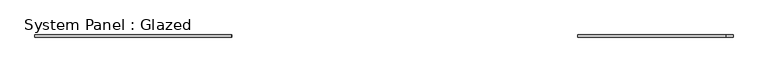
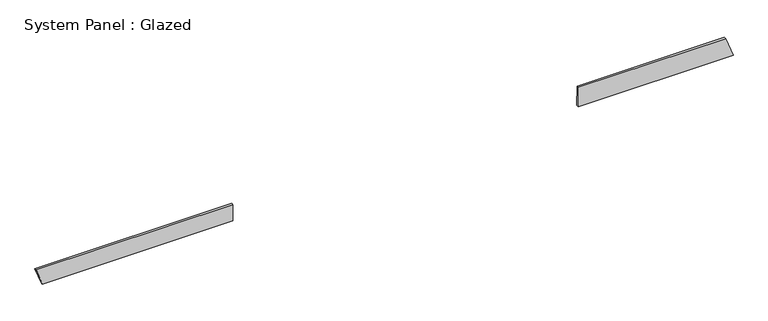
"""IFC4 building model written with IfcOpenShell, lengths in millimetres: plate geometry, System Panel : Glazed."""

from ifc_helpers import new_model, si_unit, frame, origin, place, context, project, spatial, polyline, outline, extrude, source, transform, mapped, element, save


def system_panel_glazed_ea32a12a(model_context):
    return source(origin(), model_context, "Body", "SweptSolid", [
        extrude(outline(polyline([(0.0, 2242.0624851), (0.0, 4035.4320594), (234.126736, 3950.0305658), (234.2376133, 2242.5425947), (0.0, 2242.0624851)])), frame((0.0, -49.5, 0.0), z_axis=(0.0, 1.0, 0.0), x_axis=(0.0, 0.0, 1.0)), (0.0, 0.0, 1.0), 25.0),
        extrude(outline(polyline([(0.0, -3964.1196538), (0.0, -1757.7133715), (199.142057, -1758.0632723), (199.28994, -4035.4320594), (0.0, -3964.1196538)])), frame((0.0, -49.5, 0.0), z_axis=(0.0, 1.0, 0.0), x_axis=(0.0, 0.0, 1.0)), (0.0, 0.0, 1.0), 25.0),
    ])


if __name__ == "__main__":
    model = new_model("IFC4")
    model_context = context("Model", 3, world=origin())
    ifc_project = project(units=[si_unit("LENGTHUNIT", "METRE", prefix="MILLI")], contexts=[model_context])
    site = spatial("IfcSite", under=ifc_project)
    building = spatial("IfcBuilding", under=site)
    placement = place(None, origin())
    system_panel_glazed_shape = system_panel_glazed_ea32a12a(model_context)
    element("IfcPlate", 1, ObjectType="System Panel : Glazed", at=placement, inside=building, context=model_context, shape_type="MappedRepresentation", body=[
        mapped(system_panel_glazed_shape, transform((0.0, 0.0, 0.0), x_axis=(1.0, 0.0, 0.0), y_axis=(0.0, 1.0, 0.0), z_axis=(0.0, 0.0, 1.0))),
    ])
    save(model, "model.ifc")

# Revit data of these elements
# Element 1 (IfcPlate, "System Panel : Glazed")
#   Materials on its faces: "Glass"
# Materials
#   "Glass": class "Glass", colour RGB 218 227 224, transparency 0.85, Description = "Soda Lime Glass", Cost = 0
